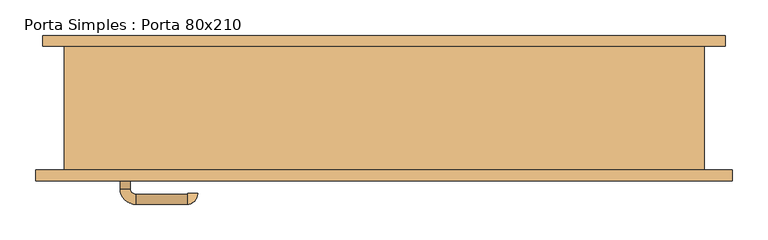
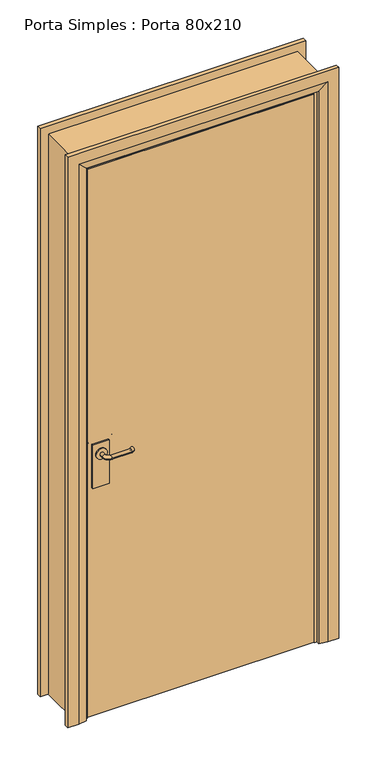
"""IFC4 building model written with IfcOpenShell, lengths in millimetres: door geometry, Porta Simples : Porta 80x210."""

from ifc_helpers import new_model, si_unit, point, frame, frame_2d, origin, place, context, project, spatial, polyline, circle_curve, ellipse_curve, trimmed, segment, composite_curve, outline, extrude, faceted_brep, source, transform, mapped, element, save
from ifc_brep_helpers import plane_surface, cylinder_surface, revolved_surface, advanced_brep


def porta_simples_porta_80x210_20d964b4(model_context):
    return source(origin(), model_context, "Body", "SolidModel", [
        extrude(outline(composite_curve([segment(trimmed(circle_curve(frame_2d((1050.0, -364.0)), 20.0), [point((1050.0, -384.0))], [point((1050.0, -344.0))], False, "CARTESIAN"), True, "CONTINUOUS"), segment(trimmed(circle_curve(frame_2d((1050.0, -364.0)), 20.0), [point((1050.0, -344.0))], [point((1050.0, -384.0))], False, "CARTESIAN"), True, "CONTINUOUS")], self_intersect=False)), frame((0.0, -46.3, 0.0), z_axis=(0.0, 1.0, 0.0), x_axis=(0.0, 0.0, 1.0)), (0.0, 0.0, 1.0), 4.5929895),
        advanced_brep(
        [(-357.0, -41.7070105, 1050.0), (-371.0, -41.7070105, 1050.0), (-357.0, -26.3, 1050.0), (-371.0, -26.3, 1050.0), (-349.0, -4.3, 1050.0), (-349.0, -18.3, 1050.0), (-277.0, -18.3, 1050.0), (-277.0, -4.3, 1050.0), (-276.0, -19.3, 1050.0), (-262.0, -19.3, 1050.0)],
        [
            (0, 1, circle_curve(frame((-364.0, -41.7070105, 1050.0), z_axis=(0.0, -1.0, 0.0), x_axis=(-1.0, 0.0, 0.0)), 7.0)),
            (1, 0, circle_curve(frame((-364.0, -41.7070105, 1050.0), z_axis=(0.0, -1.0, 0.0), x_axis=(-1.0, 0.0, 0.0)), 7.0)),
            (0, 2),
            (2, 3, circle_curve(frame((-364.0, -26.3, 1050.0), z_axis=(0.0, -1.0, 0.0), x_axis=(-1.0, 0.0, 0.0)), 7.0)),
            (3, 1),
            (3, 2, circle_curve(frame((-364.0, -26.3, 1050.0), z_axis=(0.0, -1.0, 0.0), x_axis=(-1.0, 0.0, 0.0)), 7.0)),
            (4, 3, circle_curve(frame((-349.0, -26.3, 1050.0), z_axis=(0.0, 0.0, 1.0), x_axis=(-1.0, 0.0, 0.0)), 22.0)),
            (2, 5, circle_curve(frame((-349.0, -26.3, 1050.0), z_axis=(0.0, 0.0, -1.0), x_axis=(-1.0, 0.0, 0.0)), 8.0)),
            (5, 4, circle_curve(frame((-349.0, -11.3, 1050.0), z_axis=(-1.0, 0.0, 0.0), x_axis=(0.0, 1.0, 0.0)), 7.0)),
            (4, 5, circle_curve(frame((-349.0, -11.3, 1050.0), z_axis=(-1.0, 0.0, 0.0), x_axis=(0.0, 1.0, 0.0)), 7.0)),
            (5, 6),
            (6, 7, circle_curve(frame((-277.0, -11.3, 1050.0), z_axis=(-1.0, 0.0, 0.0), x_axis=(0.0, 1.0, 0.0)), 7.0)),
            (7, 4),
            (7, 6, circle_curve(frame((-277.0, -11.3, 1050.0), z_axis=(-1.0, 0.0, 0.0), x_axis=(0.0, 1.0, 0.0)), 7.0)),
            (8, 9, circle_curve(frame((-269.0, -19.3, 1050.0), z_axis=(0.0, -1.0, 0.0), x_axis=(1.0, 0.0, 0.0)), 7.0)),
            (9, 8, circle_curve(frame((-269.0, -19.3, 1050.0), z_axis=(0.0, -1.0, 0.0), x_axis=(1.0, 0.0, 0.0)), 7.0)),
            (9, 7, circle_curve(frame((-277.0, -19.3, 1050.0), z_axis=(0.0, 0.0, 1.0), x_axis=(0.0, 1.0, 0.0)), 15.0)),
            (6, 8, circle_curve(frame((-277.0, -19.3, 1050.0), z_axis=(0.0, 0.0, -1.0), x_axis=(0.0, 1.0, 0.0)), 1.0)),
        ],
        [
            plane_surface(frame((-364.0, -41.7070105, 1050.0), z_axis=(0.0, -1.0, 0.0), x_axis=(0.0, 0.0, 1.0))),
            cylinder_surface(frame((-364.0, -41.7070105, 1050.0), z_axis=(0.0, -1.0, 0.0), x_axis=(-1.0, 0.0, 0.0)), 7.0),
            revolved_surface(trimmed(ellipse_curve(frame((-364.0, -26.3, 1050.0), z_axis=(0.0, -1.0, 0.0), x_axis=(-1.0, 0.0, 0.0)), 7.0, 7.0), [point((-357.0, -26.3, 1050.0))], [point((-371.0, -26.3, 1050.0))], True, "CARTESIAN"), (-349.0, -26.3, 1050.0), (0.0, 0.0, -1.0)),
            revolved_surface(trimmed(ellipse_curve(frame((-364.0, -26.3, 1050.0), z_axis=(0.0, -1.0, 0.0), x_axis=(-1.0, 0.0, 0.0)), 7.0, 7.0), [point((-371.0, -26.3, 1050.0))], [point((-357.0, -26.3, 1050.0))], True, "CARTESIAN"), (-349.0, -26.3, 1050.0), (0.0, 0.0, -1.0)),
            cylinder_surface(frame((-349.0, -11.3, 1050.0), z_axis=(-1.0, 0.0, 0.0), x_axis=(0.0, 1.0, 0.0)), 7.0),
            plane_surface(frame((-269.0, -19.3, 1050.0), z_axis=(0.0, -1.0, 0.0), x_axis=(0.0, 0.0, 1.0))),
            revolved_surface(trimmed(ellipse_curve(frame((-277.0, -11.3, 1050.0), z_axis=(-1.0, 0.0, 0.0), x_axis=(0.0, 1.0, 0.0)), 7.0, 7.0), [point((-277.0, -18.3, 1050.0))], [point((-277.0, -4.3, 1050.0))], True, "CARTESIAN"), (-277.0, -19.3, 1050.0), (0.0, 0.0, -1.0)),
            revolved_surface(trimmed(ellipse_curve(frame((-277.0, -11.3, 1050.0), z_axis=(-1.0, 0.0, 0.0), x_axis=(0.0, 1.0, 0.0)), 7.0, 7.0), [point((-277.0, -4.3, 1050.0))], [point((-277.0, -18.3, 1050.0))], True, "CARTESIAN"), (-277.0, -19.3, 1050.0), (0.0, 0.0, -1.0)),
        ],
        [
            (0, [[1, 2]]),
            (1, [[-1, 3, 4, 5]]),
            (1, [[-2, -5, 6, -3]]),
            (2, [[7, -4, 8, 9]]),
            (3, [[-8, -6, -7, 10]]),
            (4, [[-9, 11, 12, 13]]),
            (4, [[-10, -13, 14, -11]]),
            (5, [[15, 16]]),
            (6, [[17, -12, 18, -16]]),
            (7, [[-18, -14, -17, -15]]),
        ],
    ),
        extrude(outline(polyline([(-334.0, -52.3), (-394.0, -52.3), (-394.0, -46.3), (-334.0, -46.3), (-334.0, -52.3)])), frame((0.0, 0.0, 925.0), z_axis=(0.0, 0.0, 1.0), x_axis=(1.0, 0.0, 0.0)), (0.0, 0.0, 1.0), 165.0),
        extrude(outline(composite_curve([segment(trimmed(circle_curve(frame_2d((1050.0, -364.0)), 20.0), [point((1050.0, -384.0))], [point((1050.0, -344.0))], False, "CARTESIAN"), True, "CONTINUOUS"), segment(trimmed(circle_curve(frame_2d((1050.0, -364.0)), 20.0), [point((1050.0, -344.0))], [point((1050.0, -384.0))], False, "CARTESIAN"), True, "CONTINUOUS")], self_intersect=False)), frame((0.0, -97.8929895, 0.0), z_axis=(0.0, 1.0, 0.0), x_axis=(0.0, 0.0, 1.0)), (0.0, 0.0, 1.0), 4.5929895),
        advanced_brep(
        [(-357.0, -97.8929895, 1050.0), (-371.0, -97.8929895, 1050.0), (-371.0, -113.3, 1050.0), (-357.0, -113.3, 1050.0), (-349.0, -135.3, 1050.0), (-349.0, -121.3, 1050.0), (-277.0, -135.3, 1050.0), (-277.0, -121.3, 1050.0), (-276.0, -120.3, 1050.0), (-262.0, -120.3, 1050.0)],
        [
            (0, 1, circle_curve(frame((-364.0, -97.8929895, 1050.0), z_axis=(0.0, 1.0, 0.0), x_axis=(-1.0, 0.0, 0.0)), 7.0)),
            (1, 0, circle_curve(frame((-364.0, -97.8929895, 1050.0), z_axis=(0.0, 1.0, 0.0), x_axis=(-1.0, 0.0, 0.0)), 7.0)),
            (1, 2),
            (2, 3, circle_curve(frame((-364.0, -113.3, 1050.0), z_axis=(0.0, 1.0, 0.0), x_axis=(-1.0, 0.0, 0.0)), 7.0)),
            (3, 0),
            (3, 2, circle_curve(frame((-364.0, -113.3, 1050.0), z_axis=(0.0, 1.0, 0.0), x_axis=(-1.0, 0.0, 0.0)), 7.0)),
            (4, 5, circle_curve(frame((-349.0, -128.3, 1050.0), z_axis=(-1.0, 0.0, 0.0), x_axis=(0.0, -1.0, 0.0)), 7.0)),
            (5, 3, circle_curve(frame((-349.0, -113.3, 1050.0), z_axis=(0.0, 0.0, -1.0), x_axis=(-1.0, 0.0, 0.0)), 8.0)),
            (2, 4, circle_curve(frame((-349.0, -113.3, 1050.0), z_axis=(0.0, 0.0, 1.0), x_axis=(-1.0, 0.0, 0.0)), 22.0)),
            (5, 4, circle_curve(frame((-349.0, -128.3, 1050.0), z_axis=(-1.0, 0.0, 0.0), x_axis=(0.0, -1.0, 0.0)), 7.0)),
            (4, 6),
            (6, 7, circle_curve(frame((-277.0, -128.3, 1050.0), z_axis=(-1.0, 0.0, 0.0), x_axis=(0.0, -1.0, 0.0)), 7.0)),
            (7, 5),
            (7, 6, circle_curve(frame((-277.0, -128.3, 1050.0), z_axis=(-1.0, 0.0, 0.0), x_axis=(0.0, -1.0, 0.0)), 7.0)),
            (8, 9, circle_curve(frame((-269.0, -120.3, 1050.0), z_axis=(0.0, 1.0, 0.0), x_axis=(1.0, 0.0, 0.0)), 7.0)),
            (9, 8, circle_curve(frame((-269.0, -120.3, 1050.0), z_axis=(0.0, 1.0, 0.0), x_axis=(1.0, 0.0, 0.0)), 7.0)),
            (8, 7, circle_curve(frame((-277.0, -120.3, 1050.0), z_axis=(0.0, 0.0, -1.0), x_axis=(0.0, -1.0, 0.0)), 1.0)),
            (6, 9, circle_curve(frame((-277.0, -120.3, 1050.0), z_axis=(0.0, 0.0, 1.0), x_axis=(0.0, -1.0, 0.0)), 15.0)),
        ],
        [
            plane_surface(frame((-364.0, -97.8929895, 1050.0), z_axis=(0.0, 1.0, 0.0), x_axis=(0.0, 0.0, 1.0))),
            cylinder_surface(frame((-364.0, -97.8929895, 1050.0), z_axis=(0.0, 1.0, 0.0), x_axis=(-1.0, 0.0, 0.0)), 7.0),
            revolved_surface(trimmed(ellipse_curve(frame((-364.0, -113.3, 1050.0), z_axis=(0.0, -1.0, 0.0), x_axis=(-1.0, 0.0, 0.0)), 7.0, 7.0), [point((-357.0, -113.3, 1050.0))], [point((-371.0, -113.3, 1050.0))], True, "CARTESIAN"), (-349.0, -113.3, 1050.0), (0.0, 0.0, -1.0)),
            revolved_surface(trimmed(ellipse_curve(frame((-364.0, -113.3, 1050.0), z_axis=(0.0, -1.0, 0.0), x_axis=(-1.0, 0.0, 0.0)), 7.0, 7.0), [point((-371.0, -113.3, 1050.0))], [point((-357.0, -113.3, 1050.0))], True, "CARTESIAN"), (-349.0, -113.3, 1050.0), (0.0, 0.0, -1.0)),
            cylinder_surface(frame((-349.0, -128.3, 1050.0), z_axis=(-1.0, 0.0, 0.0), x_axis=(0.0, -1.0, 0.0)), 7.0),
            plane_surface(frame((-269.0, -120.3, 1050.0), z_axis=(0.0, 1.0, 0.0), x_axis=(0.0, 0.0, 1.0))),
            revolved_surface(trimmed(ellipse_curve(frame((-277.0, -128.3, 1050.0), z_axis=(1.0, 0.0, 0.0), x_axis=(0.0, -1.0, 0.0)), 7.0, 7.0), [point((-277.0, -121.3, 1050.0))], [point((-277.0, -135.3, 1050.0))], True, "CARTESIAN"), (-277.0, -120.3, 1050.0), (0.0, 0.0, -1.0)),
            revolved_surface(trimmed(ellipse_curve(frame((-277.0, -128.3, 1050.0), z_axis=(1.0, 0.0, 0.0), x_axis=(0.0, -1.0, 0.0)), 7.0, 7.0), [point((-277.0, -135.3, 1050.0))], [point((-277.0, -121.3, 1050.0))], True, "CARTESIAN"), (-277.0, -120.3, 1050.0), (0.0, 0.0, -1.0)),
        ],
        [
            (0, [[1, 2]]),
            (1, [[3, 4, 5, -2]]),
            (1, [[-5, 6, -3, -1]]),
            (2, [[7, 8, -4, 9]]),
            (3, [[10, -9, -6, -8]]),
            (4, [[11, 12, 13, -7]]),
            (4, [[-13, 14, -11, -10]]),
            (5, [[15, 16]]),
            (6, [[-15, 17, -12, 18]]),
            (7, [[-16, -18, -14, -17]]),
        ],
    ),
        extrude(outline(polyline([(-334.0, -87.3), (-334.0, -93.3), (-394.0, -93.3), (-394.0, -87.3), (-334.0, -87.3)])), frame((0.0, 0.0, 925.0), z_axis=(0.0, 0.0, 1.0), x_axis=(1.0, 0.0, 0.0)), (0.0, 0.0, 1.0), 165.0),
        extrude(outline(polyline([(408.0, -52.3), (408.0, -87.3), (-408.0, -87.3), (-408.0, -52.3), (408.0, -52.3)])), frame((0.0, 0.0, 53.0), z_axis=(0.0, 0.0, 1.0), x_axis=(1.0, 0.0, 0.0)), (0.0, 0.0, 1.0), 2094.0),
        faceted_brep([(480.0, 87.3, 50.0), (410.0, 87.3, 50.0), (410.0, 97.3, 50.0), (440.0, 102.3, 50.0), (480.0, 102.3, 50.0), (480.0, 102.3, 2220.0), (480.0, 87.3, 2220.0), (440.0, 102.3, 2180.0), (-440.0, 102.3, 2180.0), (-440.0, 102.3, 50.0), (-480.0, 102.3, 50.0), (-480.0, 102.3, 2220.0), (410.0, 97.3, 2150.0), (410.0, 87.3, 2150.0), (-480.0, 87.3, 2220.0), (-480.0, 87.3, 50.0), (-410.0, 87.3, 50.0), (-410.0, 87.3, 2150.0), (-410.0, 97.3, 50.0), (-410.0, 97.3, 2150.0)], [[[0, 1, 2, 3, 4]], [[4, 5, 6, 0]], [[3, 7, 8, 9, 10, 11, 5, 4]], [[2, 12, 7, 3]], [[1, 13, 12, 2]], [[0, 6, 14, 15, 16, 17, 13, 1]], [[17, 16, 18, 19]], [[15, 10, 9, 18, 16]], [[11, 10, 15, 14]], [[19, 18, 9, 8]], [[13, 17, 19, 12]], [[5, 11, 14, 6]], [[12, 19, 8, 7]]]),
        faceted_brep([(490.0, -87.3, 50.0), (490.0, -102.3, 50.0), (450.0, -102.3, 50.0), (420.0, -97.3, 50.0), (420.0, -87.3, 50.0), (420.0, -87.3, 2160.0), (-420.0, -87.3, 2160.0), (-420.0, -87.3, 50.0), (-490.0, -87.3, 50.0), (-490.0, -87.3, 2230.0), (490.0, -87.3, 2230.0), (420.0, -97.3, 2160.0), (450.0, -102.3, 2190.0), (490.0, -102.3, 2230.0), (-490.0, -102.3, 2230.0), (-490.0, -102.3, 50.0), (-450.0, -102.3, 50.0), (-450.0, -102.3, 2190.0), (-420.0, -97.3, 50.0), (-420.0, -97.3, 2160.0)], [[[0, 1, 2, 3, 4]], [[4, 5, 6, 7, 8, 9, 10, 0]], [[3, 11, 5, 4]], [[2, 12, 11, 3]], [[1, 13, 14, 15, 16, 17, 12, 2]], [[0, 10, 13, 1]], [[9, 8, 15, 14]], [[8, 7, 18, 16, 15]], [[19, 18, 7, 6]], [[17, 16, 18, 19]], [[11, 19, 6, 5]], [[10, 9, 14, 13]], [[12, 17, 19, 11]]]),
        faceted_brep([(-410.0, -87.3, 50.0), (-450.0, -87.3, 50.0), (-450.0, 87.3, 50.0), (-400.0, 87.3, 50.0), (-400.0, -50.3, 50.0), (-410.0, -50.3, 50.0), (-410.0, -50.3, 2150.0), (-410.0, -87.3, 2150.0), (-400.0, -50.3, 2140.0), (-400.0, 87.3, 2140.0), (-450.0, 87.3, 2190.0), (-450.0, -87.3, 2190.0), (410.0, -87.3, 50.0), (410.0, -50.3, 50.0), (400.0, -50.3, 50.0), (400.0, 87.3, 50.0), (450.0, 87.3, 50.0), (450.0, -87.3, 50.0), (410.0, -87.3, 2150.0), (450.0, -87.3, 2190.0), (450.0, 87.3, 2190.0), (400.0, 87.3, 2140.0), (400.0, -50.3, 2140.0), (410.0, -50.3, 2150.0)], [[[0, 1, 2, 3, 4, 5]], [[5, 6, 7, 0]], [[4, 8, 6, 5]], [[3, 9, 8, 4]], [[2, 10, 9, 3]], [[1, 11, 10, 2]], [[0, 7, 11, 1]], [[12, 13, 14, 15, 16, 17]], [[18, 12, 17, 19]], [[19, 17, 16, 20]], [[20, 16, 15, 21]], [[21, 15, 14, 22]], [[22, 14, 13, 23]], [[23, 13, 12, 18]], [[6, 23, 18, 7]], [[8, 22, 23, 6]], [[9, 21, 22, 8]], [[10, 20, 21, 9]], [[11, 19, 20, 10]], [[7, 18, 19, 11]]]),
    ])


if __name__ == "__main__":
    model = new_model("IFC4")
    model_context = context("Model", 3, world=origin())
    ifc_project = project(units=[si_unit("LENGTHUNIT", "METRE", prefix="MILLI")], contexts=[model_context])
    site = spatial("IfcSite", under=ifc_project)
    building = spatial("IfcBuilding", under=site)
    placement = place(None, origin())
    porta_simples_porta_80x210_shape = porta_simples_porta_80x210_20d964b4(model_context)
    element("IfcDoor", 1, ObjectType="Porta Simples : Porta 80x210", at=placement, inside=building, context=model_context, shape_type="MappedRepresentation", body=[
        mapped(porta_simples_porta_80x210_shape, transform((0.0, 0.0, 0.0), x_axis=(1.0, 0.0, 0.0), y_axis=(0.0, 1.0, 0.0), z_axis=(0.0, 0.0, 1.0))),
    ])
    save(model, "model.ifc")

# Revit data of these elements
# Type "Porta Simples : Porta 80x210"
#   Type Mark = "49"
#   SINAPI = ""
#   Analytic Construction = "<Nenhum>"
#   Construction Type = "300"
#   Maçaneta [instance default] = ""
#   Fechadura [instance default] = ""
#   Vão Luz (somente para informação) = 0.78 m
#   Tolerância Folha Vertical = 0.003 m
#   Módulo Básico M = 0.10 m
#   Largura de Coordenação Modular Largura CM = 0.90 m
#   Rough Width = 0.90 m
#   Deslocamento da Horizontal da Folha = 0.00 m
#   Altura de Coordenação Modular Largura CM = 2.20 m
#   Rough Height = 2.20 m
#   Altura Nominal = 2.09 m
#   Ajuste de Coordenação Topo AC Topo = 0.01 m
#   Ajuste de Coordenação Base AC Base = 0.05 m
#   Ajuste de Coordenação AC = 0.01 m
#   Tolerância Folha Horizontal = 0.002 m
#   Largura Folha (somente para informação) = 0.796 m
#   Espessura Folha = 0.035 m
#   Maçaneta - Distância da Folha = 0.044 m
#   Maçaneta - Altura = 1.00 m
#   Largura Nominal (Largura Mn) = 0.82 m
#   Distância do Nível = 0.003 m
#   Aduela Interna Espessura = 0.04 m
#   Aduela Externa Espessura = 0.05 m
#   Altura Folha (somente para informação) = 2.075 m
#   Height = 2.14 m
#   Width = 0.88 m
#   Número de Módulos Básicos nM Largura = 9
#   Número de Módulos Básicos nM Altura = 22
#   Marco Metálico = no
#   Aduela de Madeira = no
#   Aduela Metálica de Canto = no
#   Guarnição Reta = no
#   Guarnição Chanfrada = yes
#   Batente - Material [instance default] = none
#   Painel - Material [instance default] = none
#   Model = ""
#   Function = (empty or 0)
#   Description = (empty or 0)
#   Wall Closure = (empty or 0)
#   Assembly Code = ""
# Element 1 (IfcDoor, "Porta Simples : Porta 80x210")
#   Materials on its faces: "Porta - Maçaneta"
# Materials
#   "Porta - Maçaneta": class "Diversos", colour RGB 0 0 0, transparency 0
